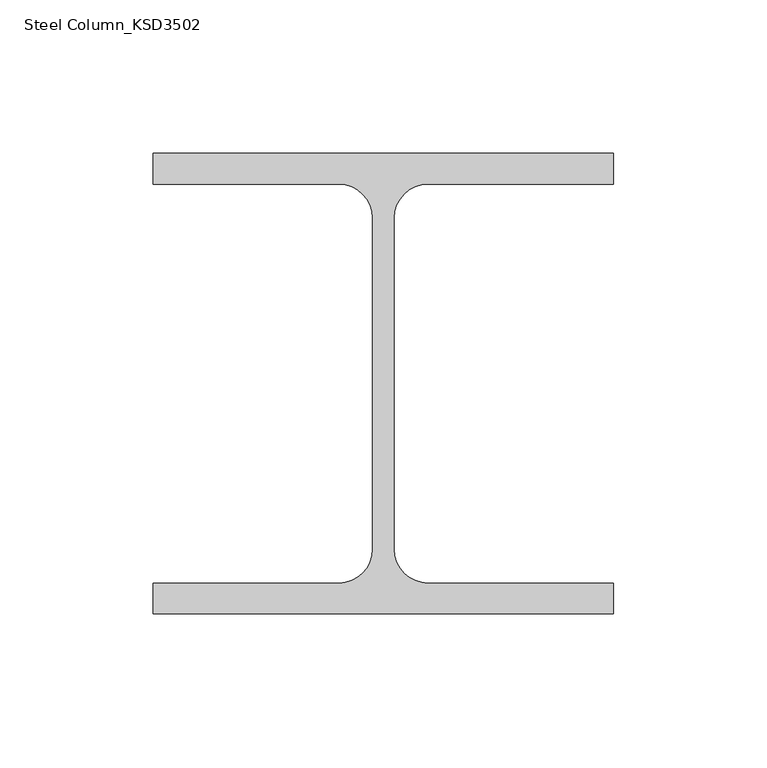
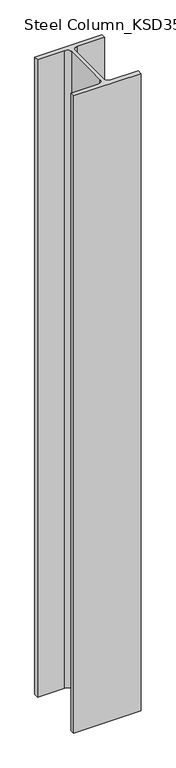
"""IFC4 building model written with IfcOpenShell, lengths in millimetres: column geometry, Steel Column_KSD3502 : H_SC_ASC_H-150×150x7x10."""

import ifcopenshell
import ifcopenshell.guid

model = None  # the IFC model being written
_history = None  # IfcOwnerHistory: only IFC2X3 demands one
_inside = {}  # id of a spatial element -> (the spatial element, [elements in it])
_under = {}  # id of a project, library or spatial element -> (it, [spatial elements below it])
_declared = {}  # id of a project -> (the project, [libraries it declares])
_typed = {}  # id of a type object -> (the type object, [elements of that type])
_made_of = {}  # id of a material, layer set ... -> (it, [elements and type objects made of it])


def new_model(schema):
    """Start an empty IFC model of exactly this schema.

    Asked for "IFC4X3", IfcOpenShell would pick the latest addendum, in which some entities
    have other attributes; the version numbers below select the first issue.
    IFC2X3 requires an IfcOwnerHistory on every rooted entity: one is made here for all.
    """
    global model, _history
    if schema == "IFC4X3":
        model = ifcopenshell.file(schema_version=(4, 3, 0, 0))
    else:
        model = ifcopenshell.file(schema=schema)
    _inside.clear()
    _under.clear()
    _declared.clear()
    _typed.clear()
    _made_of.clear()
    _history = None
    if model.schema == "IFC2X3":
        org = make("IfcOrganization", Name="unknown")
        user = make(
            "IfcPersonAndOrganization",
            ThePerson=make("IfcPerson", FamilyName="unknown"),
            TheOrganization=org,
        )
        app = make(
            "IfcApplication",
            ApplicationDeveloper=org,
            Version="unknown",
            ApplicationFullName="unknown",
            ApplicationIdentifier="unknown",
        )
        _history = make(
            "IfcOwnerHistory",
            OwningUser=user,
            OwningApplication=app,
            ChangeAction="ADDED",
            CreationDate=0,
        )
    return model


def make(cls, **values):
    """One entity of the class cls with the attributes given. An attribute that is None is left unset."""
    return model.create_entity(
        cls, **{name: value for name, value in values.items() if value is not None}
    )


def rooted(cls, **values):
    """An entity with a GlobalId (a new one), such as an element, a storey or a relation."""
    return make(cls, GlobalId=ifcopenshell.guid.new(), OwnerHistory=_history, **values)


def si_unit(unit_type, name, prefix=None):
    """IfcSIUnit, for example si_unit("LENGTHUNIT", "METRE", prefix="MILLI")."""
    return make("IfcSIUnit", UnitType=unit_type, Prefix=prefix, Name=name)


def assignment(units):
    """IfcUnitAssignment: the units of a project."""
    return None if units is None else make("IfcUnitAssignment", Units=units)


def point(xyz):
    """IfcCartesianPoint."""
    return None if xyz is None else make("IfcCartesianPoint", Coordinates=xyz)


def direction(xyz):
    """IfcDirection."""
    return None if xyz is None else make("IfcDirection", DirectionRatios=xyz)


def frame(location, z_axis=None, x_axis=None):
    """IfcAxis2Placement3D, a coordinate frame: its origin and axes. An axis left out is left unset."""
    return make(
        "IfcAxis2Placement3D",
        Location=point(location),
        Axis=direction(z_axis),
        RefDirection=direction(x_axis),
    )


def frame_2d(location, x_axis=None):
    """IfcAxis2Placement2D, a coordinate frame in the plane: its origin and x axis."""
    return make(
        "IfcAxis2Placement2D", Location=point(location), RefDirection=direction(x_axis)
    )


def origin():
    """The frame at (0, 0, 0) with its axes left unset."""
    return frame((0.0, 0.0, 0.0))


def place(relative_to, where):
    """IfcLocalPlacement: puts the frame where relative to a parent placement (None: the world)."""
    return make(
        "IfcLocalPlacement", PlacementRelTo=relative_to, RelativePlacement=where
    )


def context(
    kind, dimensions, precision=None, world=None, true_north=None, identifier=None
):
    """IfcGeometricRepresentationContext, for example the 3D "Model" context."""
    return make(
        "IfcGeometricRepresentationContext",
        ContextIdentifier=identifier,
        ContextType=kind,
        CoordinateSpaceDimension=dimensions,
        Precision=precision,
        WorldCoordinateSystem=world,
        TrueNorth=true_north,
    )


def project(units=None, contexts=None):
    """IfcProject with its units and contexts."""
    return rooted(
        "IfcProject",
        Name="project",
        RepresentationContexts=contexts,
        UnitsInContext=assignment(units),
    )


def spatial(cls, under=None, at=None, **own):
    """A site, building, storey or space (cls), placed at a placement, below another one or the project."""
    s = rooted(cls, ObjectPlacement=at, **own)
    if under is not None:
        _under.setdefault(under.id(), (under, []))[1].append(s)
    return s


def polyline(points):
    """IfcPolyline through the points."""
    return make("IfcPolyline", Points=[point(p) for p in points])


def circle_curve(where, radius):
    """IfcCircle in the frame where."""
    return make("IfcCircle", Position=where, Radius=radius)


def trimmed(basis, trim1, trim2, sense, master):
    """IfcTrimmedCurve: the piece of a basis curve between two trims."""
    return make(
        "IfcTrimmedCurve",
        BasisCurve=basis,
        Trim1=trim1,
        Trim2=trim2,
        SenseAgreement=sense,
        MasterRepresentation=master,
    )


def segment(curve, same_sense, transition):
    """IfcCompositeCurveSegment."""
    return make(
        "IfcCompositeCurveSegment",
        Transition=transition,
        SameSense=same_sense,
        ParentCurve=curve,
    )


def composite_curve(segments, self_intersect=None):
    """IfcCompositeCurve: segments joined end to end."""
    return make("IfcCompositeCurve", Segments=segments, SelfIntersect=self_intersect)


def outline(outer, holes=None, kind="AREA"):
    """IfcArbitraryClosedProfileDef: a profile drawn as a closed curve; with holes, ...WithVoids."""
    if holes is None:
        return make("IfcArbitraryClosedProfileDef", ProfileType=kind, OuterCurve=outer)
    return make(
        "IfcArbitraryProfileDefWithVoids",
        ProfileType=kind,
        OuterCurve=outer,
        InnerCurves=holes,
    )


def extrude(swept, where, along, depth):
    """IfcExtrudedAreaSolid: the profile swept, set in the frame where, extruded along a direction by depth."""
    return make(
        "IfcExtrudedAreaSolid",
        SweptArea=swept,
        Position=where,
        ExtrudedDirection=direction(along),
        Depth=depth,
    )


def shape(context_of_items, identifier, shape_type, items):
    """IfcShapeRepresentation: the items that make up one representation, for example the "Body"."""
    return make(
        "IfcShapeRepresentation",
        ContextOfItems=context_of_items,
        RepresentationIdentifier=identifier,
        RepresentationType=shape_type,
        Items=items,
    )


def source(mapping_origin, context_of_items, identifier, shape_type, items):
    """IfcRepresentationMap: a shape defined once, which mapped items show again and again."""
    return make(
        "IfcRepresentationMap",
        MappingOrigin=mapping_origin,
        MappedRepresentation=shape(context_of_items, identifier, shape_type, items),
    )


def transform(
    local_origin,
    x_axis=None,
    y_axis=None,
    z_axis=None,
    scale=None,
    scale2=None,
    scale3=None,
    uniform=True,
):
    """IfcCartesianTransformationOperator3D, or its non-uniform kind. x_axis, y_axis, z_axis: its Axis1, 2, 3."""
    if uniform:
        return make(
            "IfcCartesianTransformationOperator3D",
            Axis1=direction(x_axis),
            Axis2=direction(y_axis),
            LocalOrigin=point(local_origin),
            Scale=scale,
            Axis3=direction(z_axis),
        )
    return make(
        "IfcCartesianTransformationOperator3DnonUniform",
        Axis1=direction(x_axis),
        Axis2=direction(y_axis),
        LocalOrigin=point(local_origin),
        Scale=scale,
        Axis3=direction(z_axis),
        Scale2=scale2,
        Scale3=scale3,
    )


def mapped(mapping_source, mapping_target):
    """IfcMappedItem: shows the shape of a source again, moved by a transform."""
    return make(
        "IfcMappedItem", MappingSource=mapping_source, MappingTarget=mapping_target
    )


def made_of(thing, what):
    """Note that an element or type object is made of a material, layer set ...; save() writes the relation."""
    if what is not None:
        _made_of.setdefault(what.id(), (what, []))[1].append(thing)
    return thing


def element(
    cls,
    number,
    at=None,
    inside=None,
    cuts=None,
    type_object=None,
    material=None,
    context=None,
    identifier="Body",
    shape_type=None,
    held_by="IfcProductDefinitionShape",
    body=None,
    shapes=None,
    **own,
):
    """One element of the class cls, such as IfcWall. Its Tag is "e" and its number.

    at: its placement. inside: the storey or other place that contains it. cuts: it is an
    opening in that element (IfcRelVoidsElement). A single representation is given by context,
    identifier, shape_type and body (its items); several are given by shapes. held_by: the class
    of the entity that holds the representations. save() writes the other relations.
    """
    e = rooted(cls, Tag="e%d" % number, ObjectPlacement=at, **own)
    if body is not None:
        shapes = [shape(context, identifier, shape_type, body)]
    if shapes is not None:
        e.Representation = make(held_by, Representations=shapes)
    if inside is not None:
        _inside.setdefault(inside.id(), (inside, []))[1].append(e)
    if cuts is not None:
        rooted(
            "IfcRelVoidsElement", RelatingBuildingElement=cuts, RelatedOpeningElement=e
        )
    if type_object is not None:
        _typed.setdefault(type_object.id(), (type_object, []))[1].append(e)
    return made_of(e, material)


def aggregate(whole, parts):
    """IfcRelAggregates: a whole, such as a stair, and the parts it consists of."""
    return rooted("IfcRelAggregates", RelatingObject=whole, RelatedObjects=parts)


def save(model, path):
    """Write the relations noted so far, then the file.

    IfcRelAggregates (storeys below a building ...), IfcRelContainedInSpatialStructure (elements
    in a storey), IfcRelDefinesByType, IfcRelAssociatesMaterial and IfcRelDeclares: one each for
    every whole, place, type object, material and project.
    """
    for whole, parts in _under.values():
        aggregate(whole, parts)
    for where, things in _inside.values():
        rooted(
            "IfcRelContainedInSpatialStructure",
            RelatedElements=things,
            RelatingStructure=where,
        )
    for kind, things in _typed.values():
        rooted("IfcRelDefinesByType", RelatedObjects=things, RelatingType=kind)
    for what, things in _made_of.values():
        rooted("IfcRelAssociatesMaterial", RelatedObjects=things, RelatingMaterial=what)
    for by, libraries in _declared.values():
        rooted("IfcRelDeclares", RelatingContext=by, RelatedDefinitions=libraries)
    model.write(path)


def steel_column_ksd3502_24869f1c(model_context):
    return source(origin(), model_context, "Body", "SweptSolid", [
        extrude(outline(composite_curve([segment(polyline([(75.0, 75.0), (75.0, 65.0), (14.5, 65.0)]), True, "CONTINUOUS"), segment(trimmed(circle_curve(frame_2d((14.5, 54.0)), 11.0), [point((14.5, 65.0))], [point((3.5, 54.0))], True, "CARTESIAN"), True, "CONTINUOUS"), segment(polyline([(3.5, 54.0), (3.5, -54.0)]), True, "CONTINUOUS"), segment(trimmed(circle_curve(frame_2d((14.5, -54.0)), 11.0), [point((3.5, -54.0))], [point((14.5, -65.0))], True, "CARTESIAN"), True, "CONTINUOUS"), segment(polyline([(14.5, -65.0), (75.0, -65.0), (75.0, -75.0), (-75.0, -75.0), (-75.0, -65.0), (-14.5, -65.0)]), True, "CONTINUOUS"), segment(trimmed(circle_curve(frame_2d((-14.5, -54.0)), 11.0), [point((-14.5, -65.0))], [point((-3.5, -54.0))], True, "CARTESIAN"), True, "CONTINUOUS"), segment(polyline([(-3.5, -54.0), (-3.5, 54.0)]), True, "CONTINUOUS"), segment(trimmed(circle_curve(frame_2d((-14.5, 54.0)), 11.0), [point((-3.5, 54.0))], [point((-14.5, 65.0))], True, "CARTESIAN"), True, "CONTINUOUS"), segment(polyline([(-14.5, 65.0), (-75.0, 65.0), (-75.0, 75.0), (75.0, 75.0)]), True, "CONTINUOUS")], self_intersect=False)), frame((0.0, 0.0, 17299.9720055), z_axis=(0.0, 0.0, 1.0), x_axis=(1.0, 0.0, 0.0)), (0.0, 0.0, 1.0), 1500.0),
    ])


if __name__ == "__main__":
    model = new_model("IFC4")
    model_context = context("Model", 3, world=origin())
    ifc_project = project(units=[si_unit("LENGTHUNIT", "METRE", prefix="MILLI")], contexts=[model_context])
    site = spatial("IfcSite", under=ifc_project)
    building = spatial("IfcBuilding", under=site)
    placement = place(None, origin())
    steel_column_ksd3502_shape = steel_column_ksd3502_24869f1c(model_context)
    element("IfcColumn", 1, ObjectType="Steel Column_KSD3502 : H_SC_ASC_H-150×150x7x10", at=placement, inside=building, context=model_context, shape_type="MappedRepresentation", body=[
        mapped(steel_column_ksd3502_shape, transform((0.0, 0.0, 0.0), x_axis=(1.0, 0.0, 0.0), y_axis=(0.0, 1.0, 0.0), z_axis=(0.0, 0.0, 1.0))),
    ])
    save(model, "model.ifc")

# Revit data of these elements
# Type "Steel Column_KSD3502 : H_SC_ASC_H-150×150x7x10"
#   Width = 15.0 cm
#   Web Thickness = 0.7 cm
#   Web Fillet = 1.1 cm
#   Warping Constant = 27562.5 cm⁶
#   Torsional Moment of Inertia = 11.6007 cm⁴
#   Section Area = 40.14 cm²
#   Plastic Modulus weak axis = 115.0 cm³
#   Plastic Modulus strong axis = 246.0 cm³
#   Perimeter = 1.27 m²/m
#   Nominal Weight = 31.50 kgf/m
#   Moment of Inertia weak axis = 563.00 cm⁴
#   Moment of Inertia strong axis = 1640.00 cm⁴
#   Height = 15.0 cm
#   Flange Thickness = 1.0 cm
#   Elastic Modulus weak axis = 75.1 cm³
#   Elastic Modulus strong axis = 219.0 cm³
#   Centroid Vertical = 7.5 cm
#   Centroid Horizontal = 7.5 cm
#   Bolt Spacing = 13.97 cm
#   Structural Material [instance default] = Steel, 45-345
#   Section Name Key = ""
#   Assembly Code = ""
# Element 1 (IfcColumn, "Steel Column_KSD3502 : H_SC_ASC_H-150×150x7x10")
#   Structural Material = none
# Materials
#   "Steel, 45-345": class "Metal", colour RGB 189 187 185, transparency 0, Description = "Steel 345 MPa", Cost = 0
